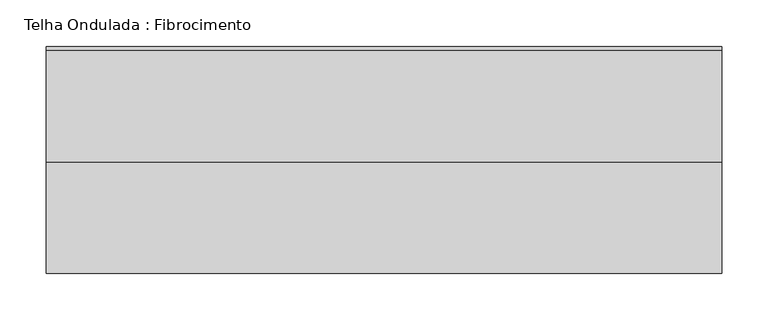
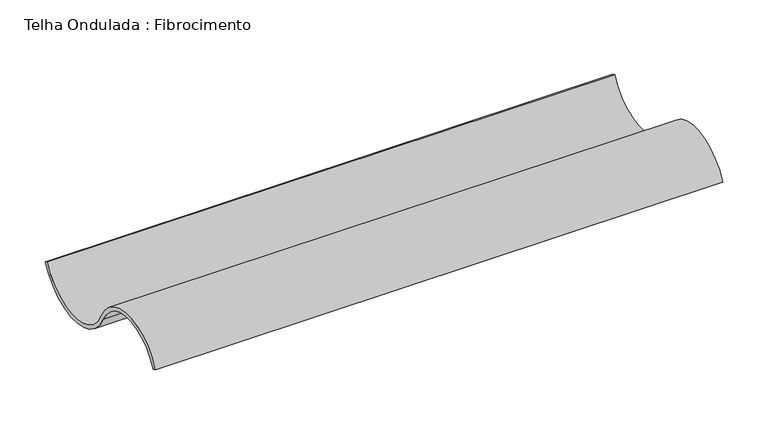
"""IFC4 building model written with IfcOpenShell, lengths in millimetres: beam geometry, Telha Ondulada : Fibrocimento."""

import ifcopenshell
import ifcopenshell.guid

model = None  # the IFC model being written
_history = None  # IfcOwnerHistory: only IFC2X3 demands one
_inside = {}  # id of a spatial element -> (the spatial element, [elements in it])
_under = {}  # id of a project, library or spatial element -> (it, [spatial elements below it])
_declared = {}  # id of a project -> (the project, [libraries it declares])
_typed = {}  # id of a type object -> (the type object, [elements of that type])
_made_of = {}  # id of a material, layer set ... -> (it, [elements and type objects made of it])


def new_model(schema):
    """Start an empty IFC model of exactly this schema.

    Asked for "IFC4X3", IfcOpenShell would pick the latest addendum, in which some entities
    have other attributes; the version numbers below select the first issue.
    IFC2X3 requires an IfcOwnerHistory on every rooted entity: one is made here for all.
    """
    global model, _history
    if schema == "IFC4X3":
        model = ifcopenshell.file(schema_version=(4, 3, 0, 0))
    else:
        model = ifcopenshell.file(schema=schema)
    _inside.clear()
    _under.clear()
    _declared.clear()
    _typed.clear()
    _made_of.clear()
    _history = None
    if model.schema == "IFC2X3":
        org = make("IfcOrganization", Name="unknown")
        user = make(
            "IfcPersonAndOrganization",
            ThePerson=make("IfcPerson", FamilyName="unknown"),
            TheOrganization=org,
        )
        app = make(
            "IfcApplication",
            ApplicationDeveloper=org,
            Version="unknown",
            ApplicationFullName="unknown",
            ApplicationIdentifier="unknown",
        )
        _history = make(
            "IfcOwnerHistory",
            OwningUser=user,
            OwningApplication=app,
            ChangeAction="ADDED",
            CreationDate=0,
        )
    return model


def make(cls, **values):
    """One entity of the class cls with the attributes given. An attribute that is None is left unset."""
    return model.create_entity(
        cls, **{name: value for name, value in values.items() if value is not None}
    )


def rooted(cls, **values):
    """An entity with a GlobalId (a new one), such as an element, a storey or a relation."""
    return make(cls, GlobalId=ifcopenshell.guid.new(), OwnerHistory=_history, **values)


def si_unit(unit_type, name, prefix=None):
    """IfcSIUnit, for example si_unit("LENGTHUNIT", "METRE", prefix="MILLI")."""
    return make("IfcSIUnit", UnitType=unit_type, Prefix=prefix, Name=name)


def assignment(units):
    """IfcUnitAssignment: the units of a project."""
    return None if units is None else make("IfcUnitAssignment", Units=units)


def point(xyz):
    """IfcCartesianPoint."""
    return None if xyz is None else make("IfcCartesianPoint", Coordinates=xyz)


def direction(xyz):
    """IfcDirection."""
    return None if xyz is None else make("IfcDirection", DirectionRatios=xyz)


def frame(location, z_axis=None, x_axis=None):
    """IfcAxis2Placement3D, a coordinate frame: its origin and axes. An axis left out is left unset."""
    return make(
        "IfcAxis2Placement3D",
        Location=point(location),
        Axis=direction(z_axis),
        RefDirection=direction(x_axis),
    )


def frame_2d(location, x_axis=None):
    """IfcAxis2Placement2D, a coordinate frame in the plane: its origin and x axis."""
    return make(
        "IfcAxis2Placement2D", Location=point(location), RefDirection=direction(x_axis)
    )


def origin():
    """The frame at (0, 0, 0) with its axes left unset."""
    return frame((0.0, 0.0, 0.0))


def place(relative_to, where):
    """IfcLocalPlacement: puts the frame where relative to a parent placement (None: the world)."""
    return make(
        "IfcLocalPlacement", PlacementRelTo=relative_to, RelativePlacement=where
    )


def context(
    kind, dimensions, precision=None, world=None, true_north=None, identifier=None
):
    """IfcGeometricRepresentationContext, for example the 3D "Model" context."""
    return make(
        "IfcGeometricRepresentationContext",
        ContextIdentifier=identifier,
        ContextType=kind,
        CoordinateSpaceDimension=dimensions,
        Precision=precision,
        WorldCoordinateSystem=world,
        TrueNorth=true_north,
    )


def project(units=None, contexts=None):
    """IfcProject with its units and contexts."""
    return rooted(
        "IfcProject",
        Name="project",
        RepresentationContexts=contexts,
        UnitsInContext=assignment(units),
    )


def spatial(cls, under=None, at=None, **own):
    """A site, building, storey or space (cls), placed at a placement, below another one or the project."""
    s = rooted(cls, ObjectPlacement=at, **own)
    if under is not None:
        _under.setdefault(under.id(), (under, []))[1].append(s)
    return s


def polyline(points):
    """IfcPolyline through the points."""
    return make("IfcPolyline", Points=[point(p) for p in points])


def circle_curve(where, radius):
    """IfcCircle in the frame where."""
    return make("IfcCircle", Position=where, Radius=radius)


def trimmed(basis, trim1, trim2, sense, master):
    """IfcTrimmedCurve: the piece of a basis curve between two trims."""
    return make(
        "IfcTrimmedCurve",
        BasisCurve=basis,
        Trim1=trim1,
        Trim2=trim2,
        SenseAgreement=sense,
        MasterRepresentation=master,
    )


def segment(curve, same_sense, transition):
    """IfcCompositeCurveSegment."""
    return make(
        "IfcCompositeCurveSegment",
        Transition=transition,
        SameSense=same_sense,
        ParentCurve=curve,
    )


def composite_curve(segments, self_intersect=None):
    """IfcCompositeCurve: segments joined end to end."""
    return make("IfcCompositeCurve", Segments=segments, SelfIntersect=self_intersect)


def outline(outer, holes=None, kind="AREA"):
    """IfcArbitraryClosedProfileDef: a profile drawn as a closed curve; with holes, ...WithVoids."""
    if holes is None:
        return make("IfcArbitraryClosedProfileDef", ProfileType=kind, OuterCurve=outer)
    return make(
        "IfcArbitraryProfileDefWithVoids",
        ProfileType=kind,
        OuterCurve=outer,
        InnerCurves=holes,
    )


def extrude(swept, where, along, depth):
    """IfcExtrudedAreaSolid: the profile swept, set in the frame where, extruded along a direction by depth."""
    return make(
        "IfcExtrudedAreaSolid",
        SweptArea=swept,
        Position=where,
        ExtrudedDirection=direction(along),
        Depth=depth,
    )


def shape(context_of_items, identifier, shape_type, items):
    """IfcShapeRepresentation: the items that make up one representation, for example the "Body"."""
    return make(
        "IfcShapeRepresentation",
        ContextOfItems=context_of_items,
        RepresentationIdentifier=identifier,
        RepresentationType=shape_type,
        Items=items,
    )


def source(mapping_origin, context_of_items, identifier, shape_type, items):
    """IfcRepresentationMap: a shape defined once, which mapped items show again and again."""
    return make(
        "IfcRepresentationMap",
        MappingOrigin=mapping_origin,
        MappedRepresentation=shape(context_of_items, identifier, shape_type, items),
    )


def transform(
    local_origin,
    x_axis=None,
    y_axis=None,
    z_axis=None,
    scale=None,
    scale2=None,
    scale3=None,
    uniform=True,
):
    """IfcCartesianTransformationOperator3D, or its non-uniform kind. x_axis, y_axis, z_axis: its Axis1, 2, 3."""
    if uniform:
        return make(
            "IfcCartesianTransformationOperator3D",
            Axis1=direction(x_axis),
            Axis2=direction(y_axis),
            LocalOrigin=point(local_origin),
            Scale=scale,
            Axis3=direction(z_axis),
        )
    return make(
        "IfcCartesianTransformationOperator3DnonUniform",
        Axis1=direction(x_axis),
        Axis2=direction(y_axis),
        LocalOrigin=point(local_origin),
        Scale=scale,
        Axis3=direction(z_axis),
        Scale2=scale2,
        Scale3=scale3,
    )


def mapped(mapping_source, mapping_target):
    """IfcMappedItem: shows the shape of a source again, moved by a transform."""
    return make(
        "IfcMappedItem", MappingSource=mapping_source, MappingTarget=mapping_target
    )


def made_of(thing, what):
    """Note that an element or type object is made of a material, layer set ...; save() writes the relation."""
    if what is not None:
        _made_of.setdefault(what.id(), (what, []))[1].append(thing)
    return thing


def element(
    cls,
    number,
    at=None,
    inside=None,
    cuts=None,
    type_object=None,
    material=None,
    context=None,
    identifier="Body",
    shape_type=None,
    held_by="IfcProductDefinitionShape",
    body=None,
    shapes=None,
    **own,
):
    """One element of the class cls, such as IfcWall. Its Tag is "e" and its number.

    at: its placement. inside: the storey or other place that contains it. cuts: it is an
    opening in that element (IfcRelVoidsElement). A single representation is given by context,
    identifier, shape_type and body (its items); several are given by shapes. held_by: the class
    of the entity that holds the representations. save() writes the other relations.
    """
    e = rooted(cls, Tag="e%d" % number, ObjectPlacement=at, **own)
    if body is not None:
        shapes = [shape(context, identifier, shape_type, body)]
    if shapes is not None:
        e.Representation = make(held_by, Representations=shapes)
    if inside is not None:
        _inside.setdefault(inside.id(), (inside, []))[1].append(e)
    if cuts is not None:
        rooted(
            "IfcRelVoidsElement", RelatingBuildingElement=cuts, RelatedOpeningElement=e
        )
    if type_object is not None:
        _typed.setdefault(type_object.id(), (type_object, []))[1].append(e)
    return made_of(e, material)


def aggregate(whole, parts):
    """IfcRelAggregates: a whole, such as a stair, and the parts it consists of."""
    return rooted("IfcRelAggregates", RelatingObject=whole, RelatedObjects=parts)


def save(model, path):
    """Write the relations noted so far, then the file.

    IfcRelAggregates (storeys below a building ...), IfcRelContainedInSpatialStructure (elements
    in a storey), IfcRelDefinesByType, IfcRelAssociatesMaterial and IfcRelDeclares: one each for
    every whole, place, type object, material and project.
    """
    for whole, parts in _under.values():
        aggregate(whole, parts)
    for where, things in _inside.values():
        rooted(
            "IfcRelContainedInSpatialStructure",
            RelatedElements=things,
            RelatingStructure=where,
        )
    for kind, things in _typed.values():
        rooted("IfcRelDefinesByType", RelatedObjects=things, RelatingType=kind)
    for what, things in _made_of.values():
        rooted("IfcRelAssociatesMaterial", RelatedObjects=things, RelatingMaterial=what)
    for by, libraries in _declared.values():
        rooted("IfcRelDeclares", RelatingContext=by, RelatedDefinitions=libraries)
    model.write(path)


def telha_ondulada_fibrocimento_963230a9(model_context):
    return source(origin(), model_context, "Body", "SweptSolid", [
        extrude(outline(composite_curve([segment(trimmed(circle_curve(frame_2d((68.3970135, 71.7939461)), 66.7939461), [point((8.3970135, 42.4437972))], [point((128.3970135, 42.4437972))], True, "CARTESIAN"), True, "CONTINUOUS"), segment(polyline([(128.3970135, 42.4437972), (132.8884385, 40.2467307)]), True, "CONTINUOUS"), segment(trimmed(circle_curve(frame_2d((68.3970135, 71.7939461)), 71.7939461), [point((132.8884385, 40.2467307))], [point((3.9055884, 40.2467307))], False, "CARTESIAN"), True, "CONTINUOUS"), segment(trimmed(circle_curve(frame_2d((-51.6029865, 13.0936483)), 61.7939461), [point((3.9055884, 40.2467307))], [point((-107.1115615, 40.2467307))], True, "CARTESIAN"), True, "CONTINUOUS"), segment(polyline([(-107.1115615, 40.2467307), (-111.6029865, 42.4437972)]), True, "CONTINUOUS"), segment(trimmed(circle_curve(frame_2d((-51.6029865, 13.0936483)), 66.7939461), [point((-111.6029865, 42.4437972))], [point((8.3970135, 42.4437972))], False, "CARTESIAN"), True, "CONTINUOUS")], self_intersect=False)), frame((-362.9289365, 0.0, 0.0), z_axis=(1.0, 0.0, 0.0), x_axis=(0.0, 1.0, 0.0)), (0.0, 0.0, 1.0), 725.8578731),
    ])


if __name__ == "__main__":
    model = new_model("IFC4")
    model_context = context("Model", 3, world=origin())
    ifc_project = project(units=[si_unit("LENGTHUNIT", "METRE", prefix="MILLI")], contexts=[model_context])
    site = spatial("IfcSite", under=ifc_project)
    building = spatial("IfcBuilding", under=site)
    placement = place(None, origin())
    telha_ondulada_fibrocimento_shape = telha_ondulada_fibrocimento_963230a9(model_context)
    element("IfcBeam", 1, ObjectType="Telha Ondulada : Fibrocimento", at=placement, inside=building, context=model_context, shape_type="MappedRepresentation", body=[
        mapped(telha_ondulada_fibrocimento_shape, transform((0.0, 0.0, 0.0), x_axis=(1.0, 0.0, 0.0), y_axis=(0.0, 1.0, 0.0), z_axis=(0.0, 0.0, 1.0))),
    ])
    save(model, "model.ifc")

# Revit data of these elements
# Type "Telha Ondulada : Fibrocimento"
#   Description = "TELHA ONDULADA FIBROCIMENTO"
#   Cost = 5
#   Length [instance default] = 1.524 m
#   b = 0.07 m
#   h = 0.16 m
#   Structural Material = .TELHA DE FIBROCIMENTO
#   Assembly Code = ""
# Element 1 (IfcBeam, "Telha Ondulada : Fibrocimento")
#   Materials on its faces: ".TELHA DE FIBROCIMENTO"
# Materials
#   ".TELHA DE FIBROCIMENTO": class "CC_TELHADO", colour RGB 77 77 76, transparency 0, Description = "TELHA ONDULADA FIBROCIMENTO", Cost = 0
